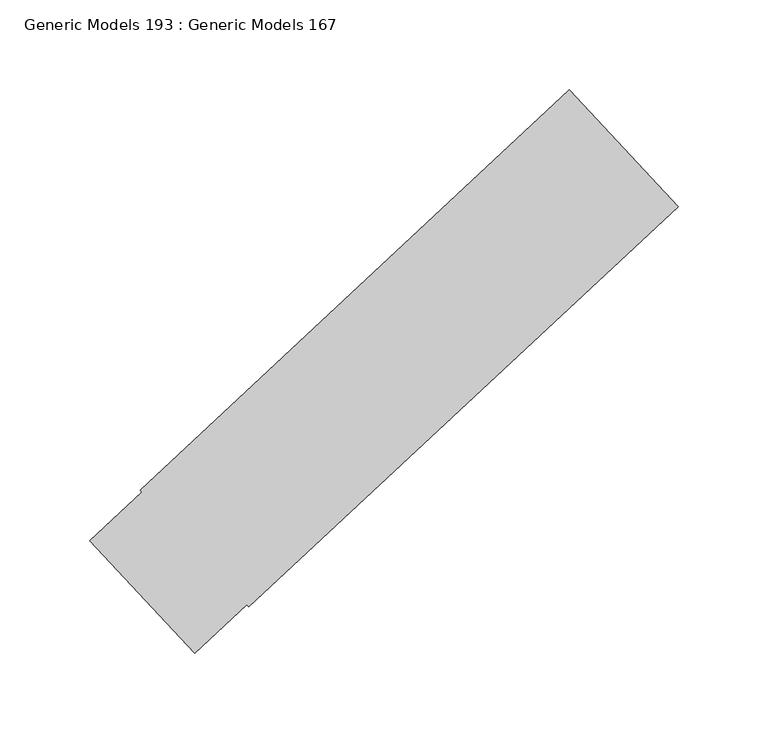
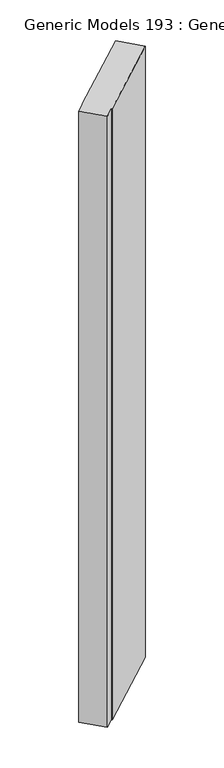
"""IFC4 building model written with IfcOpenShell, lengths in millimetres: proxy geometry, Generic Models 193 : Generic Models 167."""

from ifc_helpers import new_model, si_unit, origin, origin_with_axes, place, context, project, spatial, polyline, outline, extrude, source, transform, mapped, element, save


def generic_models_193_generic_models_167_a93b3b67(model_context):
    return source(origin(), model_context, "Body", "SweptSolid", [
        extrude(outline(polyline([(59501.993454, 4543.6894938), (59562.6231082, 4478.6721497), (59323.6888765, 4255.8623741), (59322.6062041, 4257.0233981), (59293.5806041, 4229.9565882), (59235.1162947, 4292.6518843), (59264.1418947, 4319.7186942), (59263.0592223, 4320.8797182), (59501.993454, 4543.6894938)])), origin_with_axes(), (0.0, 0.0, 1.0), 2133.6),
    ])


if __name__ == "__main__":
    model = new_model("IFC4")
    model_context = context("Model", 3, world=origin())
    ifc_project = project(units=[si_unit("LENGTHUNIT", "METRE", prefix="MILLI")], contexts=[model_context])
    site = spatial("IfcSite", under=ifc_project)
    building = spatial("IfcBuilding", under=site)
    placement = place(None, origin())
    generic_models_193_generic_models_167_shape = generic_models_193_generic_models_167_a93b3b67(model_context)
    element("IfcBuildingElementProxy", 1, Name="Generic Models 193 : Generic Models 167", ObjectType="Generic Models 193 : Generic Models 167", at=placement, inside=building, context=model_context, shape_type="MappedRepresentation", body=[
        mapped(generic_models_193_generic_models_167_shape, transform((0.0, 0.0, 0.0), x_axis=(1.0, 0.0, 0.0), y_axis=(0.0, 1.0, 0.0), z_axis=(0.0, 0.0, 1.0))),
    ])
    save(model, "model.ifc")

# Revit data of these elements
# Element 1 (IfcBuildingElementProxy, "Generic Models 193 : Generic Models 167")
#   Materials on its faces: "METAL STUDS (MATCH EXISTING SIZE/GAUGE/SPACING)"
# Materials
#   "METAL STUDS (MATCH EXISTING SIZE/GAUGE/SPACING)": class "Unassigned", colour RGB 210 209 208, transparency 0, Keynote = "M05121300.02", Cost = 0
